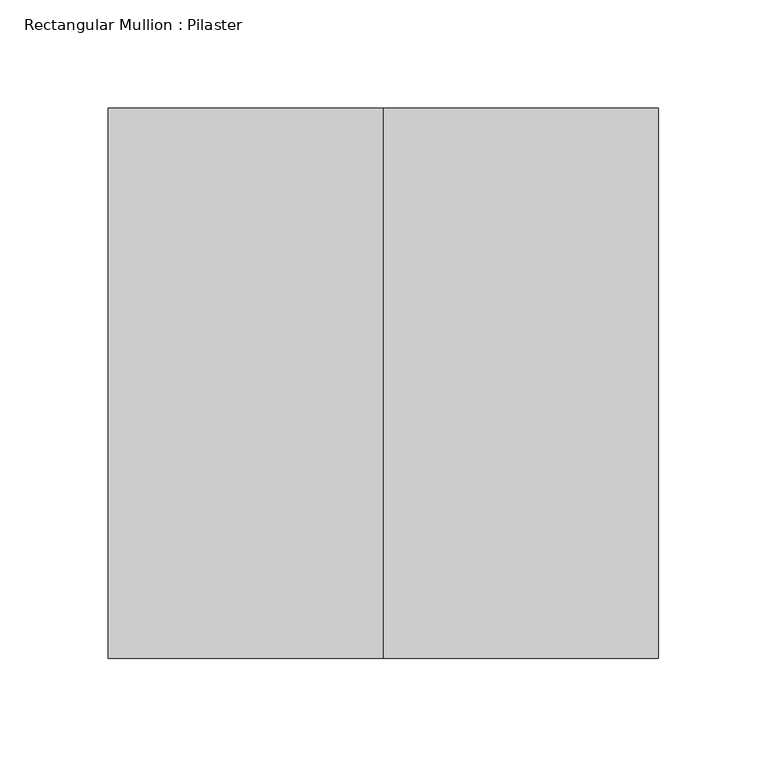
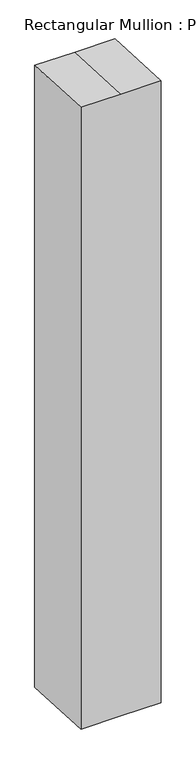
"""IFC4 building model written with IfcOpenShell, lengths in millimetres: member geometry, Rectangular Mullion : Pilaster."""

import ifcopenshell
import ifcopenshell.guid

model = None  # the IFC model being written
_history = None  # IfcOwnerHistory: only IFC2X3 demands one
_inside = {}  # id of a spatial element -> (the spatial element, [elements in it])
_under = {}  # id of a project, library or spatial element -> (it, [spatial elements below it])
_declared = {}  # id of a project -> (the project, [libraries it declares])
_typed = {}  # id of a type object -> (the type object, [elements of that type])
_made_of = {}  # id of a material, layer set ... -> (it, [elements and type objects made of it])


def new_model(schema):
    """Start an empty IFC model of exactly this schema.

    Asked for "IFC4X3", IfcOpenShell would pick the latest addendum, in which some entities
    have other attributes; the version numbers below select the first issue.
    IFC2X3 requires an IfcOwnerHistory on every rooted entity: one is made here for all.
    """
    global model, _history
    if schema == "IFC4X3":
        model = ifcopenshell.file(schema_version=(4, 3, 0, 0))
    else:
        model = ifcopenshell.file(schema=schema)
    _inside.clear()
    _under.clear()
    _declared.clear()
    _typed.clear()
    _made_of.clear()
    _history = None
    if model.schema == "IFC2X3":
        org = make("IfcOrganization", Name="unknown")
        user = make(
            "IfcPersonAndOrganization",
            ThePerson=make("IfcPerson", FamilyName="unknown"),
            TheOrganization=org,
        )
        app = make(
            "IfcApplication",
            ApplicationDeveloper=org,
            Version="unknown",
            ApplicationFullName="unknown",
            ApplicationIdentifier="unknown",
        )
        _history = make(
            "IfcOwnerHistory",
            OwningUser=user,
            OwningApplication=app,
            ChangeAction="ADDED",
            CreationDate=0,
        )
    return model


def make(cls, **values):
    """One entity of the class cls with the attributes given. An attribute that is None is left unset."""
    return model.create_entity(
        cls, **{name: value for name, value in values.items() if value is not None}
    )


def rooted(cls, **values):
    """An entity with a GlobalId (a new one), such as an element, a storey or a relation."""
    return make(cls, GlobalId=ifcopenshell.guid.new(), OwnerHistory=_history, **values)


def si_unit(unit_type, name, prefix=None):
    """IfcSIUnit, for example si_unit("LENGTHUNIT", "METRE", prefix="MILLI")."""
    return make("IfcSIUnit", UnitType=unit_type, Prefix=prefix, Name=name)


def assignment(units):
    """IfcUnitAssignment: the units of a project."""
    return None if units is None else make("IfcUnitAssignment", Units=units)


def point(xyz):
    """IfcCartesianPoint."""
    return None if xyz is None else make("IfcCartesianPoint", Coordinates=xyz)


def direction(xyz):
    """IfcDirection."""
    return None if xyz is None else make("IfcDirection", DirectionRatios=xyz)


def frame(location, z_axis=None, x_axis=None):
    """IfcAxis2Placement3D, a coordinate frame: its origin and axes. An axis left out is left unset."""
    return make(
        "IfcAxis2Placement3D",
        Location=point(location),
        Axis=direction(z_axis),
        RefDirection=direction(x_axis),
    )


def origin():
    """The frame at (0, 0, 0) with its axes left unset."""
    return frame((0.0, 0.0, 0.0))


def place(relative_to, where):
    """IfcLocalPlacement: puts the frame where relative to a parent placement (None: the world)."""
    return make(
        "IfcLocalPlacement", PlacementRelTo=relative_to, RelativePlacement=where
    )


def context(
    kind, dimensions, precision=None, world=None, true_north=None, identifier=None
):
    """IfcGeometricRepresentationContext, for example the 3D "Model" context."""
    return make(
        "IfcGeometricRepresentationContext",
        ContextIdentifier=identifier,
        ContextType=kind,
        CoordinateSpaceDimension=dimensions,
        Precision=precision,
        WorldCoordinateSystem=world,
        TrueNorth=true_north,
    )


def project(units=None, contexts=None):
    """IfcProject with its units and contexts."""
    return rooted(
        "IfcProject",
        Name="project",
        RepresentationContexts=contexts,
        UnitsInContext=assignment(units),
    )


def spatial(cls, under=None, at=None, **own):
    """A site, building, storey or space (cls), placed at a placement, below another one or the project."""
    s = rooted(cls, ObjectPlacement=at, **own)
    if under is not None:
        _under.setdefault(under.id(), (under, []))[1].append(s)
    return s


def faces_of(points, faces, orient=None, outer=None):
    """IfcFace entities. A face is a list of loops; a loop is a list of indices into points, from 0.

    orient and outer hold one flag for each loop. By default every Orientation is true, the
    first loop of a face is its IfcFaceOuterBound and the others are IfcFaceBound.
    """
    made = []
    for i, loops in enumerate(faces):
        bounds = []
        for j, loop in enumerate(loops):
            is_outer = j == 0 if outer is None else outer[i][j]
            bounds.append(
                make(
                    "IfcFaceOuterBound" if is_outer else "IfcFaceBound",
                    Bound=make("IfcPolyLoop", Polygon=[points[k] for k in loop]),
                    Orientation=True if orient is None else orient[i][j],
                )
            )
        made.append(make("IfcFace", Bounds=bounds))
    return made


def faceted_brep(points, faces, orient=None, outer=None, voids=None):
    """IfcFacetedBrep: a solid bounded by flat faces; with voids (closed shells), ...WithVoids."""
    shared = [point(p) for p in points]
    hull = make("IfcClosedShell", CfsFaces=faces_of(shared, faces, orient, outer))
    if voids is None:
        return make("IfcFacetedBrep", Outer=hull)
    return make(
        "IfcFacetedBrepWithVoids",
        Outer=hull,
        Voids=[
            make(cls, CfsFaces=faces_of(shared, fs, o, b)) for cls, fs, o, b in voids
        ],
    )


def shape(context_of_items, identifier, shape_type, items):
    """IfcShapeRepresentation: the items that make up one representation, for example the "Body"."""
    return make(
        "IfcShapeRepresentation",
        ContextOfItems=context_of_items,
        RepresentationIdentifier=identifier,
        RepresentationType=shape_type,
        Items=items,
    )


def source(mapping_origin, context_of_items, identifier, shape_type, items):
    """IfcRepresentationMap: a shape defined once, which mapped items show again and again."""
    return make(
        "IfcRepresentationMap",
        MappingOrigin=mapping_origin,
        MappedRepresentation=shape(context_of_items, identifier, shape_type, items),
    )


def transform(
    local_origin,
    x_axis=None,
    y_axis=None,
    z_axis=None,
    scale=None,
    scale2=None,
    scale3=None,
    uniform=True,
):
    """IfcCartesianTransformationOperator3D, or its non-uniform kind. x_axis, y_axis, z_axis: its Axis1, 2, 3."""
    if uniform:
        return make(
            "IfcCartesianTransformationOperator3D",
            Axis1=direction(x_axis),
            Axis2=direction(y_axis),
            LocalOrigin=point(local_origin),
            Scale=scale,
            Axis3=direction(z_axis),
        )
    return make(
        "IfcCartesianTransformationOperator3DnonUniform",
        Axis1=direction(x_axis),
        Axis2=direction(y_axis),
        LocalOrigin=point(local_origin),
        Scale=scale,
        Axis3=direction(z_axis),
        Scale2=scale2,
        Scale3=scale3,
    )


def mapped(mapping_source, mapping_target):
    """IfcMappedItem: shows the shape of a source again, moved by a transform."""
    return make(
        "IfcMappedItem", MappingSource=mapping_source, MappingTarget=mapping_target
    )


def made_of(thing, what):
    """Note that an element or type object is made of a material, layer set ...; save() writes the relation."""
    if what is not None:
        _made_of.setdefault(what.id(), (what, []))[1].append(thing)
    return thing


def element(
    cls,
    number,
    at=None,
    inside=None,
    cuts=None,
    type_object=None,
    material=None,
    context=None,
    identifier="Body",
    shape_type=None,
    held_by="IfcProductDefinitionShape",
    body=None,
    shapes=None,
    **own,
):
    """One element of the class cls, such as IfcWall. Its Tag is "e" and its number.

    at: its placement. inside: the storey or other place that contains it. cuts: it is an
    opening in that element (IfcRelVoidsElement). A single representation is given by context,
    identifier, shape_type and body (its items); several are given by shapes. held_by: the class
    of the entity that holds the representations. save() writes the other relations.
    """
    e = rooted(cls, Tag="e%d" % number, ObjectPlacement=at, **own)
    if body is not None:
        shapes = [shape(context, identifier, shape_type, body)]
    if shapes is not None:
        e.Representation = make(held_by, Representations=shapes)
    if inside is not None:
        _inside.setdefault(inside.id(), (inside, []))[1].append(e)
    if cuts is not None:
        rooted(
            "IfcRelVoidsElement", RelatingBuildingElement=cuts, RelatedOpeningElement=e
        )
    if type_object is not None:
        _typed.setdefault(type_object.id(), (type_object, []))[1].append(e)
    return made_of(e, material)


def aggregate(whole, parts):
    """IfcRelAggregates: a whole, such as a stair, and the parts it consists of."""
    return rooted("IfcRelAggregates", RelatingObject=whole, RelatedObjects=parts)


def save(model, path):
    """Write the relations noted so far, then the file.

    IfcRelAggregates (storeys below a building ...), IfcRelContainedInSpatialStructure (elements
    in a storey), IfcRelDefinesByType, IfcRelAssociatesMaterial and IfcRelDeclares: one each for
    every whole, place, type object, material and project.
    """
    for whole, parts in _under.values():
        aggregate(whole, parts)
    for where, things in _inside.values():
        rooted(
            "IfcRelContainedInSpatialStructure",
            RelatedElements=things,
            RelatingStructure=where,
        )
    for kind, things in _typed.values():
        rooted("IfcRelDefinesByType", RelatedObjects=things, RelatingType=kind)
    for what, things in _made_of.values():
        rooted("IfcRelAssociatesMaterial", RelatedObjects=things, RelatingMaterial=what)
    for by, libraries in _declared.values():
        rooted("IfcRelDeclares", RelatingContext=by, RelatedDefinitions=libraries)
    model.write(path)


def rectangular_mullion_pilaster_8c912226(model_context):
    return source(origin(), model_context, "Body", "Brep", [
        faceted_brep([(-127.0, 127.0, -7.074079), (0.0, 127.0, -7.074079), (127.0, 127.0, -7.074079), (127.0, 127.0, -2087.9711982), (0.0, 127.0, -2087.9711982), (-127.0, 127.0, -2087.9711982), (-127.0, -127.0, 6.2374969), (-127.0, -127.0, -2074.6596223), (127.0, -127.0, 6.2374969), (0.0, -127.0, 6.2374969), (0.0, -127.0, -2074.6596223), (127.0, -127.0, -2074.6596223)], [[[0, 1, 2, 3, 4, 5]], [[6, 0, 5, 7]], [[8, 9, 6, 7, 10, 11]], [[2, 8, 11, 3]], [[2, 1, 9, 8]], [[1, 0, 6, 9]], [[3, 11, 10, 4]], [[10, 7, 5, 4]]]),
    ])


if __name__ == "__main__":
    model = new_model("IFC4")
    model_context = context("Model", 3, world=origin())
    ifc_project = project(units=[si_unit("LENGTHUNIT", "METRE", prefix="MILLI")], contexts=[model_context])
    site = spatial("IfcSite", under=ifc_project)
    building = spatial("IfcBuilding", under=site)
    placement = place(None, origin())
    rectangular_mullion_pilaster_shape = rectangular_mullion_pilaster_8c912226(model_context)
    element("IfcMember", 1, ObjectType="Rectangular Mullion : Pilaster", at=placement, inside=building, context=model_context, shape_type="MappedRepresentation", body=[
        mapped(rectangular_mullion_pilaster_shape, transform((0.0, 0.0, 0.0), x_axis=(1.0, 0.0, 0.0), y_axis=(0.0, 1.0, 0.0), z_axis=(0.0, 0.0, 1.0))),
    ])
    save(model, "model.ifc")

# Revit data of these elements
# Type "Rectangular Mullion : Pilaster"
#   built-in parameter 1007304 = 0.833333 (stored number, unit not read)
#   built-in parameter 1007301 = 0.416667 (stored number, unit not read)
#   built-in parameter 1007300 = 0.416667 (stored number, unit not read)
# Element 1 (IfcMember, "Rectangular Mullion : Pilaster")
#   Materials on its faces: "Aluminum"
# Materials
#   "Aluminum": class "Metal", colour RGB 247 247 247, transparency 0, Description = "Aluminum 6061", Cost = 0
